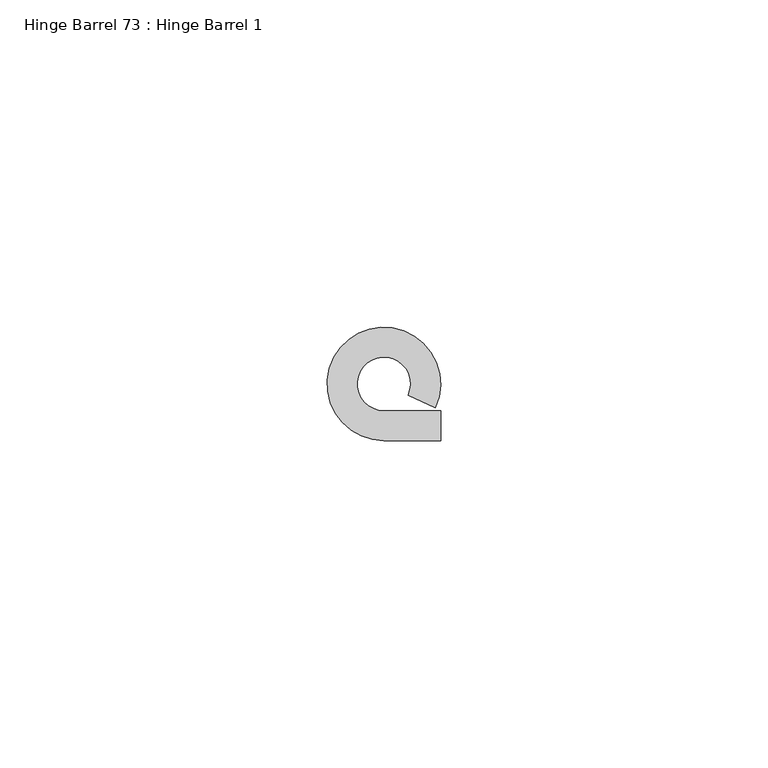
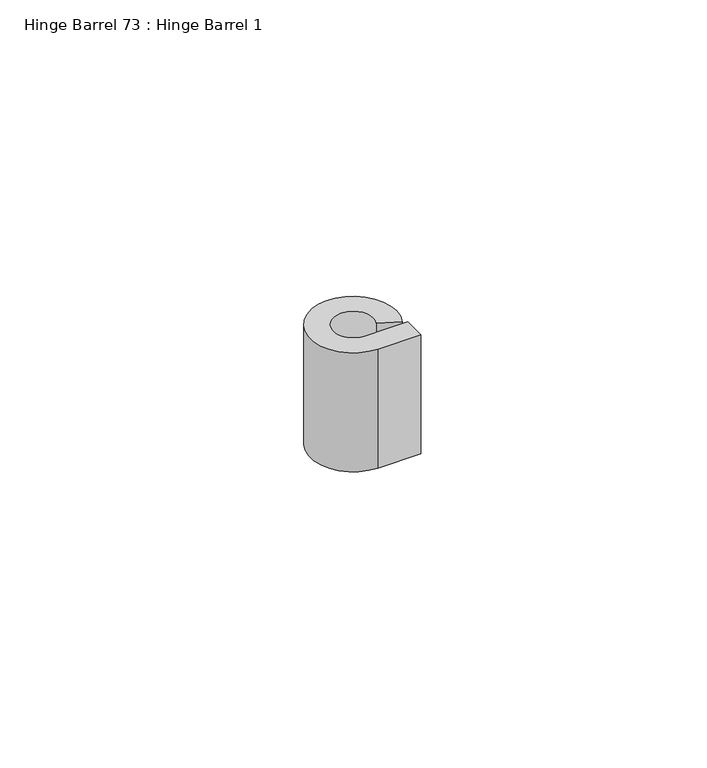
"""IFC4 building model written with IfcOpenShell, lengths in millimetres: proxy geometry, Hinge Barrel 73 : Hinge Barrel 1."""

from ifc_helpers import new_model, si_unit, point, frame, frame_2d, origin, place, context, project, spatial, polyline, circle_curve, trimmed, segment, composite_curve, outline, extrude, source, transform, mapped, element, save


def hinge_barrel_73_hinge_barrel_1_117a87e6(model_context):
    return source(origin(), model_context, "Body", "SweptSolid", [
        extrude(outline(composite_curve([segment(polyline([(587323.2214739, -531780.6943841), (587327.7934739, -531780.6943841), (587327.7934739, -531785.2584466), (587319.1320739, -531785.2584466)]), True, "CONTINUOUS"), segment(trimmed(circle_curve(frame_2d((587319.1320739, -531776.6049841)), 8.6534625), [point((587319.1320739, -531785.2584466))], [point((587326.986084, -531780.2377433))], False, "CARTESIAN"), True, "CONTINUOUS"), segment(polyline([(587326.986084, -531780.2377433), (587322.8436736, -531778.321731)]), True, "CONTINUOUS"), segment(trimmed(circle_curve(frame_2d((587319.1320739, -531776.6049841)), 4.0894), [point((587322.8436736, -531778.321731))], [point((587319.1320739, -531780.6943841))], True, "CARTESIAN"), True, "CONTINUOUS"), segment(polyline([(587319.1320739, -531780.6943841), (587323.2214739, -531780.6943841)]), True, "CONTINUOUS")], self_intersect=False)), frame((0.0, 0.0, 311.15), z_axis=(0.0, 0.0, 1.0), x_axis=(1.0, 0.0, 0.0)), (0.0, 0.0, 1.0), 25.4),
    ])


if __name__ == "__main__":
    model = new_model("IFC4")
    model_context = context("Model", 3, world=origin())
    ifc_project = project(units=[si_unit("LENGTHUNIT", "METRE", prefix="MILLI")], contexts=[model_context])
    site = spatial("IfcSite", under=ifc_project)
    building = spatial("IfcBuilding", under=site)
    placement = place(None, origin())
    hinge_barrel_73_hinge_barrel_1_shape = hinge_barrel_73_hinge_barrel_1_117a87e6(model_context)
    element("IfcBuildingElementProxy", 1, Name="Hinge Barrel 73 : Hinge Barrel 1", ObjectType="Hinge Barrel 73 : Hinge Barrel 1", at=placement, inside=building, context=model_context, shape_type="MappedRepresentation", body=[
        mapped(hinge_barrel_73_hinge_barrel_1_shape, transform((0.0, 0.0, 0.0), x_axis=(1.0, 0.0, 0.0), y_axis=(0.0, 1.0, 0.0), z_axis=(0.0, 0.0, 1.0))),
    ])
    save(model, "model.ifc")

# Revit data of these elements
# Element 1 (IfcBuildingElementProxy, "Hinge Barrel 73 : Hinge Barrel 1")
#   Materials on its faces: "6\"X6\" WELD-ON STL BUTT HINGE"
# Materials
#   "6\"X6\" WELD-ON STL BUTT HINGE": class "Metal", colour RGB 189 187 185, transparency 0, Description = "Carbon steel", Cost = 0
